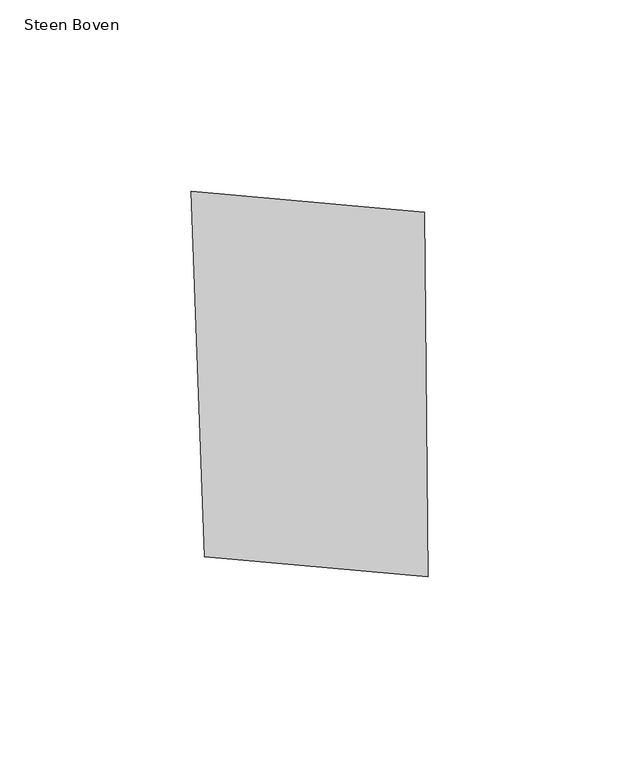
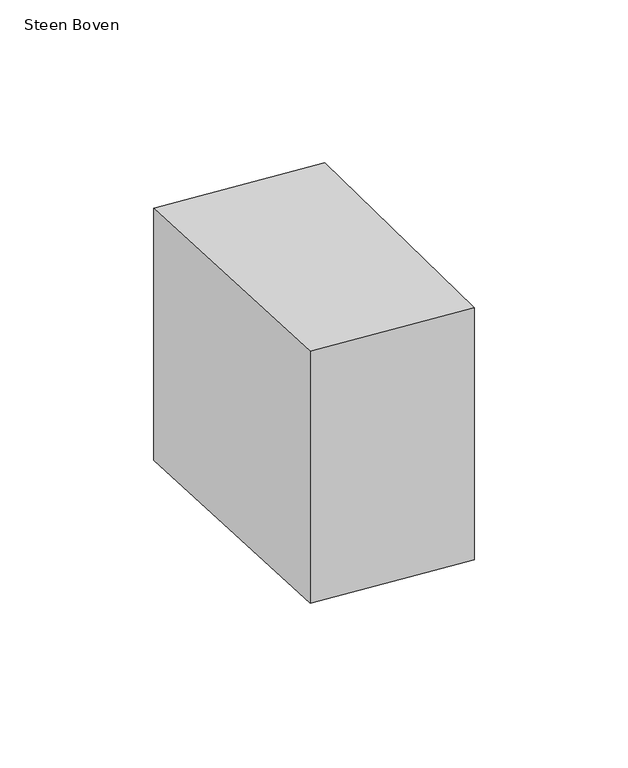
"""IFC4 building model written with IfcOpenShell, lengths in millimetres: proxy geometry, 00_GMA_steen_versie_4 : Steen Boven."""

from ifc_helpers import new_model, si_unit, origin, origin_with_axes, place, context, project, spatial, polyline, outline, extrude, source, transform, mapped, element, save


def steen_boven_d4ebafc0(model_context):
    return source(origin(), model_context, "Body", "SweptSolid", [
        extrude(outline(polyline([(100.0965651, 119.2936937), (101.0027724, 23.7980781), (42.5285842, 29.0717828), (38.9175964, 124.8257073), (100.0965651, 119.2936937)])), origin_with_axes(), (0.0, 0.0, 1.0), 100.0),
    ])


if __name__ == "__main__":
    model = new_model("IFC4")
    model_context = context("Model", 3, world=origin())
    ifc_project = project(units=[si_unit("LENGTHUNIT", "METRE", prefix="MILLI")], contexts=[model_context])
    site = spatial("IfcSite", under=ifc_project)
    building = spatial("IfcBuilding", under=site)
    placement = place(None, origin())
    steen_boven_shape = steen_boven_d4ebafc0(model_context)
    element("IfcBuildingElementProxy", 1, Name="00_GMA_steen_versie_4 : Steen Boven", ObjectType="00_GMA_steen_versie_4 : Steen Boven", at=placement, inside=building, context=model_context, shape_type="MappedRepresentation", body=[
        mapped(steen_boven_shape, transform((0.0, 0.0, 0.0), x_axis=(1.0, 0.0, 0.0), y_axis=(0.0, 1.0, 0.0), z_axis=(0.0, 0.0, 1.0))),
    ])
    save(model, "model.ifc")

# Revit data of these elements
# Type "00_GMA_steen_versie_4 : Steen Boven"
#   StootVoegHalfBoven [instance default] = 5 mm
#   StootVoegHalf [instance default] = 5 mm
#   StootVoegBreedteOnder = 10 mm
#   StootVoegBreedteBoven = 10 mm
#   Steendikte = 100 mm
#   LintVoegOnderHalf = 5 mm
#   LintVoegOnder = 10 mm
#   LintVoegBovenHalf = 0 mm
#   LintVoegBoven = 0 mm
#   materiaal = none
#   MateriaalVoeg = none
#   Default Elevation = 0
